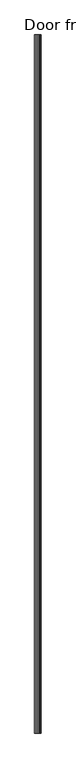
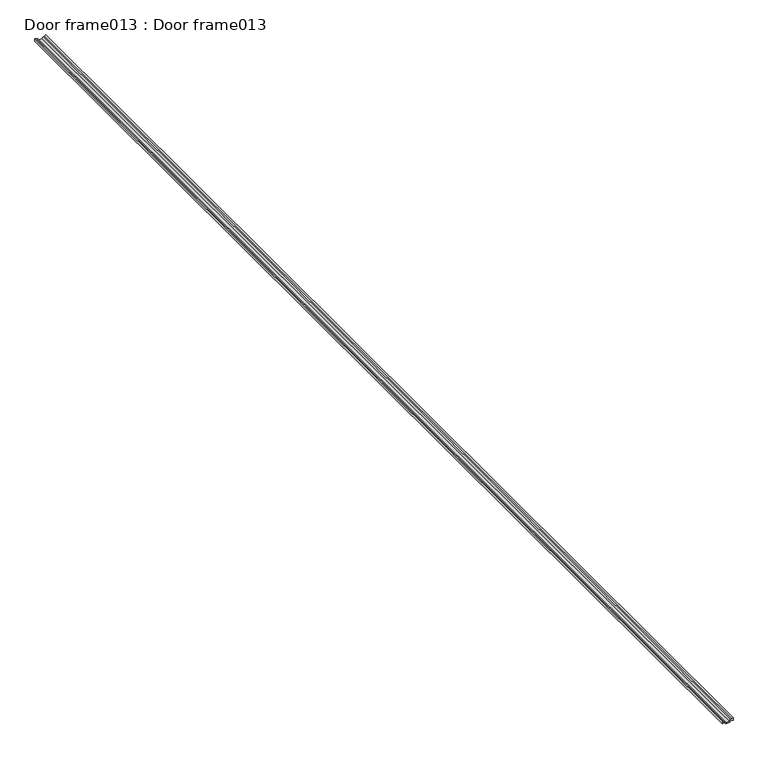
"""IFC4 building model written with IfcOpenShell, lengths in millimetres: proxy geometry, Door frame013 : Door frame013."""

from ifc_helpers import new_model, si_unit, frame, origin, place, context, project, spatial, polyline, outline, extrude, source, transform, mapped, element, save


def door_frame013_door_frame013_088115ce(model_context):
    return source(origin(), model_context, "Body", "SweptSolid", [
        extrude(outline(polyline([(36596.1835829, 15554.7629668), (36596.1835829, 15556.3015659), (36595.1059519, 15558.7219647), (36599.8429954, 15558.7219647), (36598.3174519, 15556.0796459), (36598.3174519, 15554.3038786), (36595.2518099, 15552.157293), (36595.2518099, 15546.8085492), (36598.3174519, 15544.6619636), (36598.3174519, 15542.8861964), (36599.8429954, 15540.2438775), (36595.1059519, 15540.2438775), (36596.1835829, 15542.6642763), (36596.1835829, 15544.2028754), (36593.6518099, 15545.975642), (36593.6518099, 15552.9902003), (36596.1835829, 15554.7629668)])), frame((0.0, -1052.8906567, 0.0), z_axis=(0.0, 1.0, 0.0), x_axis=(0.0, 0.0, 1.0)), (0.0, 0.0, 1.0), 1999.85),
    ])


if __name__ == "__main__":
    model = new_model("IFC4")
    model_context = context("Model", 3, world=origin())
    ifc_project = project(units=[si_unit("LENGTHUNIT", "METRE", prefix="MILLI")], contexts=[model_context])
    site = spatial("IfcSite", under=ifc_project)
    building = spatial("IfcBuilding", under=site)
    placement = place(None, origin())
    door_frame013_door_frame013_shape = door_frame013_door_frame013_088115ce(model_context)
    element("IfcBuildingElementProxy", 1, Name="Door frame013 : Door frame013", ObjectType="Door frame013 : Door frame013", at=placement, inside=building, context=model_context, shape_type="MappedRepresentation", body=[
        mapped(door_frame013_door_frame013_shape, transform((0.0, 0.0, 0.0), x_axis=(1.0, 0.0, 0.0), y_axis=(0.0, 1.0, 0.0), z_axis=(0.0, 0.0, 1.0))),
    ])
    save(model, "model.ifc")

# Revit data of these elements
# Type "Door frame013 : Door frame013"
#   NameOverride = "Door frame013"
# Element 1 (IfcBuildingElementProxy, "Door frame013 : Door frame013")
#   Materials on its faces: "FLEETWOOD SERIES T-3200 SINGLE SWING DOOR FRAME"
# Materials
#   "FLEETWOOD SERIES T-3200 SINGLE SWING DOOR FRAME": class "Unassigned", colour RGB 128 128 128, transparency 0, Cost = 0
